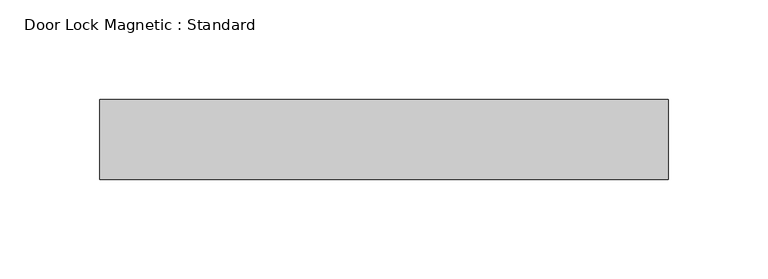
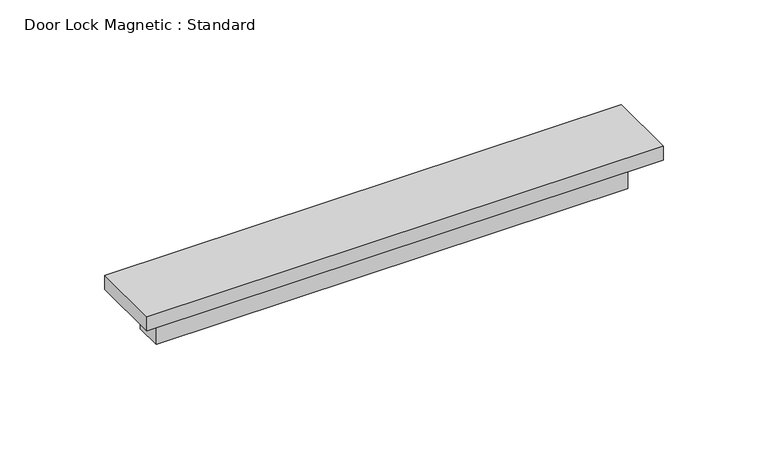
"""IFC4 building model written with IfcOpenShell, lengths in millimetres: proxy geometry, Door Lock Magnetic : Standard."""

from ifc_helpers import new_model, si_unit, frame, origin, origin_with_axes, place, context, project, spatial, polyline, outline, extrude, source, transform, mapped, element, save


def door_lock_magnetic_standard_083446a8(model_context):
    return source(origin(), model_context, "Body", "SweptSolid", [
        extrude(outline(polyline([(142.5, -40.0), (-142.5, -40.0), (-142.5, 0.0), (142.5, 0.0), (142.5, -40.0)])), origin_with_axes(), (0.0, 0.0, 1.0), 8.0),
        extrude(outline(polyline([(130.0, -27.5), (-130.0, -27.5), (-130.0, -12.5), (130.0, -12.5), (130.0, -27.5)])), frame((0.0, 0.0, -20.0), z_axis=(0.0, 0.0, 1.0), x_axis=(1.0, 0.0, 0.0)), (0.0, 0.0, 1.0), 20.0),
    ])


if __name__ == "__main__":
    model = new_model("IFC4")
    model_context = context("Model", 3, world=origin())
    ifc_project = project(units=[si_unit("LENGTHUNIT", "METRE", prefix="MILLI")], contexts=[model_context])
    site = spatial("IfcSite", under=ifc_project)
    building = spatial("IfcBuilding", under=site)
    placement = place(None, origin())
    door_lock_magnetic_standard_shape = door_lock_magnetic_standard_083446a8(model_context)
    element("IfcBuildingElementProxy", 1, Name="Door Lock Magnetic : Standard", ObjectType="Door Lock Magnetic : Standard", at=placement, inside=building, context=model_context, shape_type="MappedRepresentation", body=[
        mapped(door_lock_magnetic_standard_shape, transform((0.0, 0.0, 0.0), x_axis=(1.0, 0.0, 0.0), y_axis=(0.0, 1.0, 0.0), z_axis=(0.0, 0.0, 1.0))),
    ])
    save(model, "model.ifc")

# Revit data of these elements
# Type "Door Lock Magnetic : Standard"
#   Type Mark = "Door Lock Magnetic"
#   Classification.OmniClass.23.Number = "23-29 13 00"
#   Classification.OmniClass.23.Description = "Security Access Controls"
#   COBie.Type.CreatedBy = "info@mma.ie"
#   COBie.Type.CreatedOn = "2017-07-26T09:12:44"
#   COBie.Type.Name = "Door Lock Magnetic"
#   COBie.Type.Category = "23-29 13 00 : Security Access Controls"
#   COBie.Type.Description = "Door Lock Magnetic_Standard"
#   COBie.Type.AssetType = "Fixed"
#   COBie.Type.Manufacturer = ""
#   COBie.Type.ModelNumber = ""
#   COBie.Type.ModelReference = ""
#   COBie.Type.Color = "Stainless Steel"
#   Units = "Volts"
#   Keynote = "28 13 00.B"
#   COBie.Type.ReplacementCost = 0
#   Default Elevation = 1200 mm
#   DML_Width = 285 mm
#   DML_Height = 40 mm
#   DML_Depth = 28 mm
#   COBie.Type = yes
#   URL = ""
#   Model = ""
#   Manufacturer = ""
